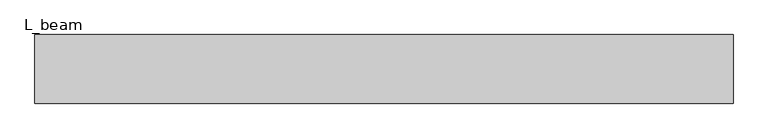
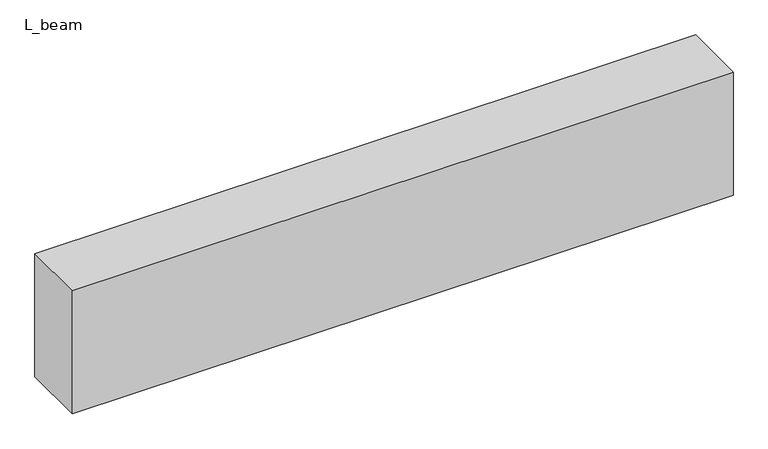
"""IFC4 building model written with IfcOpenShell, lengths in millimetres: beam geometry, 混凝土 - 矩形梁 : L_beam."""

import ifcopenshell
import ifcopenshell.guid

model = None  # the IFC model being written
_history = None  # IfcOwnerHistory: only IFC2X3 demands one
_inside = {}  # id of a spatial element -> (the spatial element, [elements in it])
_under = {}  # id of a project, library or spatial element -> (it, [spatial elements below it])
_declared = {}  # id of a project -> (the project, [libraries it declares])
_typed = {}  # id of a type object -> (the type object, [elements of that type])
_made_of = {}  # id of a material, layer set ... -> (it, [elements and type objects made of it])


def new_model(schema):
    """Start an empty IFC model of exactly this schema.

    Asked for "IFC4X3", IfcOpenShell would pick the latest addendum, in which some entities
    have other attributes; the version numbers below select the first issue.
    IFC2X3 requires an IfcOwnerHistory on every rooted entity: one is made here for all.
    """
    global model, _history
    if schema == "IFC4X3":
        model = ifcopenshell.file(schema_version=(4, 3, 0, 0))
    else:
        model = ifcopenshell.file(schema=schema)
    _inside.clear()
    _under.clear()
    _declared.clear()
    _typed.clear()
    _made_of.clear()
    _history = None
    if model.schema == "IFC2X3":
        org = make("IfcOrganization", Name="unknown")
        user = make(
            "IfcPersonAndOrganization",
            ThePerson=make("IfcPerson", FamilyName="unknown"),
            TheOrganization=org,
        )
        app = make(
            "IfcApplication",
            ApplicationDeveloper=org,
            Version="unknown",
            ApplicationFullName="unknown",
            ApplicationIdentifier="unknown",
        )
        _history = make(
            "IfcOwnerHistory",
            OwningUser=user,
            OwningApplication=app,
            ChangeAction="ADDED",
            CreationDate=0,
        )
    return model


def make(cls, **values):
    """One entity of the class cls with the attributes given. An attribute that is None is left unset."""
    return model.create_entity(
        cls, **{name: value for name, value in values.items() if value is not None}
    )


def rooted(cls, **values):
    """An entity with a GlobalId (a new one), such as an element, a storey or a relation."""
    return make(cls, GlobalId=ifcopenshell.guid.new(), OwnerHistory=_history, **values)


def si_unit(unit_type, name, prefix=None):
    """IfcSIUnit, for example si_unit("LENGTHUNIT", "METRE", prefix="MILLI")."""
    return make("IfcSIUnit", UnitType=unit_type, Prefix=prefix, Name=name)


def assignment(units):
    """IfcUnitAssignment: the units of a project."""
    return None if units is None else make("IfcUnitAssignment", Units=units)


def point(xyz):
    """IfcCartesianPoint."""
    return None if xyz is None else make("IfcCartesianPoint", Coordinates=xyz)


def direction(xyz):
    """IfcDirection."""
    return None if xyz is None else make("IfcDirection", DirectionRatios=xyz)


def frame(location, z_axis=None, x_axis=None):
    """IfcAxis2Placement3D, a coordinate frame: its origin and axes. An axis left out is left unset."""
    return make(
        "IfcAxis2Placement3D",
        Location=point(location),
        Axis=direction(z_axis),
        RefDirection=direction(x_axis),
    )


def origin():
    """The frame at (0, 0, 0) with its axes left unset."""
    return frame((0.0, 0.0, 0.0))


def place(relative_to, where):
    """IfcLocalPlacement: puts the frame where relative to a parent placement (None: the world)."""
    return make(
        "IfcLocalPlacement", PlacementRelTo=relative_to, RelativePlacement=where
    )


def context(
    kind, dimensions, precision=None, world=None, true_north=None, identifier=None
):
    """IfcGeometricRepresentationContext, for example the 3D "Model" context."""
    return make(
        "IfcGeometricRepresentationContext",
        ContextIdentifier=identifier,
        ContextType=kind,
        CoordinateSpaceDimension=dimensions,
        Precision=precision,
        WorldCoordinateSystem=world,
        TrueNorth=true_north,
    )


def project(units=None, contexts=None):
    """IfcProject with its units and contexts."""
    return rooted(
        "IfcProject",
        Name="project",
        RepresentationContexts=contexts,
        UnitsInContext=assignment(units),
    )


def spatial(cls, under=None, at=None, **own):
    """A site, building, storey or space (cls), placed at a placement, below another one or the project."""
    s = rooted(cls, ObjectPlacement=at, **own)
    if under is not None:
        _under.setdefault(under.id(), (under, []))[1].append(s)
    return s


def polyline(points):
    """IfcPolyline through the points."""
    return make("IfcPolyline", Points=[point(p) for p in points])


def outline(outer, holes=None, kind="AREA"):
    """IfcArbitraryClosedProfileDef: a profile drawn as a closed curve; with holes, ...WithVoids."""
    if holes is None:
        return make("IfcArbitraryClosedProfileDef", ProfileType=kind, OuterCurve=outer)
    return make(
        "IfcArbitraryProfileDefWithVoids",
        ProfileType=kind,
        OuterCurve=outer,
        InnerCurves=holes,
    )


def extrude(swept, where, along, depth):
    """IfcExtrudedAreaSolid: the profile swept, set in the frame where, extruded along a direction by depth."""
    return make(
        "IfcExtrudedAreaSolid",
        SweptArea=swept,
        Position=where,
        ExtrudedDirection=direction(along),
        Depth=depth,
    )


def shape(context_of_items, identifier, shape_type, items):
    """IfcShapeRepresentation: the items that make up one representation, for example the "Body"."""
    return make(
        "IfcShapeRepresentation",
        ContextOfItems=context_of_items,
        RepresentationIdentifier=identifier,
        RepresentationType=shape_type,
        Items=items,
    )


def source(mapping_origin, context_of_items, identifier, shape_type, items):
    """IfcRepresentationMap: a shape defined once, which mapped items show again and again."""
    return make(
        "IfcRepresentationMap",
        MappingOrigin=mapping_origin,
        MappedRepresentation=shape(context_of_items, identifier, shape_type, items),
    )


def transform(
    local_origin,
    x_axis=None,
    y_axis=None,
    z_axis=None,
    scale=None,
    scale2=None,
    scale3=None,
    uniform=True,
):
    """IfcCartesianTransformationOperator3D, or its non-uniform kind. x_axis, y_axis, z_axis: its Axis1, 2, 3."""
    if uniform:
        return make(
            "IfcCartesianTransformationOperator3D",
            Axis1=direction(x_axis),
            Axis2=direction(y_axis),
            LocalOrigin=point(local_origin),
            Scale=scale,
            Axis3=direction(z_axis),
        )
    return make(
        "IfcCartesianTransformationOperator3DnonUniform",
        Axis1=direction(x_axis),
        Axis2=direction(y_axis),
        LocalOrigin=point(local_origin),
        Scale=scale,
        Axis3=direction(z_axis),
        Scale2=scale2,
        Scale3=scale3,
    )


def mapped(mapping_source, mapping_target):
    """IfcMappedItem: shows the shape of a source again, moved by a transform."""
    return make(
        "IfcMappedItem", MappingSource=mapping_source, MappingTarget=mapping_target
    )


def made_of(thing, what):
    """Note that an element or type object is made of a material, layer set ...; save() writes the relation."""
    if what is not None:
        _made_of.setdefault(what.id(), (what, []))[1].append(thing)
    return thing


def element(
    cls,
    number,
    at=None,
    inside=None,
    cuts=None,
    type_object=None,
    material=None,
    context=None,
    identifier="Body",
    shape_type=None,
    held_by="IfcProductDefinitionShape",
    body=None,
    shapes=None,
    **own,
):
    """One element of the class cls, such as IfcWall. Its Tag is "e" and its number.

    at: its placement. inside: the storey or other place that contains it. cuts: it is an
    opening in that element (IfcRelVoidsElement). A single representation is given by context,
    identifier, shape_type and body (its items); several are given by shapes. held_by: the class
    of the entity that holds the representations. save() writes the other relations.
    """
    e = rooted(cls, Tag="e%d" % number, ObjectPlacement=at, **own)
    if body is not None:
        shapes = [shape(context, identifier, shape_type, body)]
    if shapes is not None:
        e.Representation = make(held_by, Representations=shapes)
    if inside is not None:
        _inside.setdefault(inside.id(), (inside, []))[1].append(e)
    if cuts is not None:
        rooted(
            "IfcRelVoidsElement", RelatingBuildingElement=cuts, RelatedOpeningElement=e
        )
    if type_object is not None:
        _typed.setdefault(type_object.id(), (type_object, []))[1].append(e)
    return made_of(e, material)


def aggregate(whole, parts):
    """IfcRelAggregates: a whole, such as a stair, and the parts it consists of."""
    return rooted("IfcRelAggregates", RelatingObject=whole, RelatedObjects=parts)


def save(model, path):
    """Write the relations noted so far, then the file.

    IfcRelAggregates (storeys below a building ...), IfcRelContainedInSpatialStructure (elements
    in a storey), IfcRelDefinesByType, IfcRelAssociatesMaterial and IfcRelDeclares: one each for
    every whole, place, type object, material and project.
    """
    for whole, parts in _under.values():
        aggregate(whole, parts)
    for where, things in _inside.values():
        rooted(
            "IfcRelContainedInSpatialStructure",
            RelatedElements=things,
            RelatingStructure=where,
        )
    for kind, things in _typed.values():
        rooted("IfcRelDefinesByType", RelatedObjects=things, RelatingType=kind)
    for what, things in _made_of.values():
        rooted("IfcRelAssociatesMaterial", RelatedObjects=things, RelatingMaterial=what)
    for by, libraries in _declared.values():
        rooted("IfcRelDeclares", RelatingContext=by, RelatedDefinitions=libraries)
    model.write(path)


def l_beam_cf5e2ff1(model_context):
    return source(origin(), model_context, "Body", "SweptSolid", [
        extrude(outline(polyline([(1526.0, 150.0), (1526.0, -150.0), (-1526.0, -150.0), (-1526.0, 150.0), (1526.0, 150.0)])), frame((0.0, 0.0, -300.0), z_axis=(0.0, 0.0, 1.0), x_axis=(1.0, 0.0, 0.0)), (0.0, 0.0, 1.0), 600.0),
    ])


if __name__ == "__main__":
    model = new_model("IFC4")
    model_context = context("Model", 3, world=origin())
    ifc_project = project(units=[si_unit("LENGTHUNIT", "METRE", prefix="MILLI")], contexts=[model_context])
    site = spatial("IfcSite", under=ifc_project)
    building = spatial("IfcBuilding", under=site)
    placement = place(None, origin())
    l_beam_shape = l_beam_cf5e2ff1(model_context)
    element("IfcBeam", 1, ObjectType="混凝土 - 矩形梁 : L_beam", at=placement, inside=building, context=model_context, shape_type="MappedRepresentation", body=[
        mapped(l_beam_shape, transform((0.0, 0.0, 0.0), x_axis=(1.0, 0.0, 0.0), y_axis=(0.0, 1.0, 0.0), z_axis=(0.0, 0.0, 1.0))),
    ])
    save(model, "model.ifc")

# Revit data of these elements
# Type "混凝土 - 矩形梁 : L_beam"
#   Length [instance default] = 1524 mm
#   b = 300 mm
#   h = 600 mm
#   Structural Material [instance default] = none
#   Assembly Code = ""
